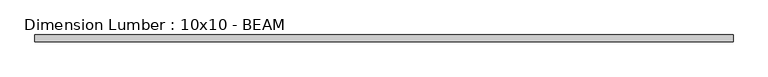
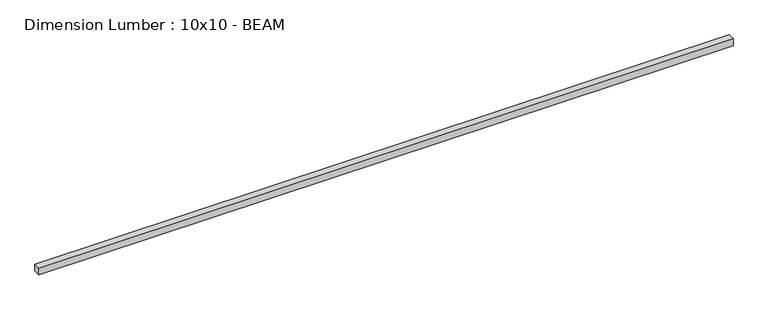
"""IFC4 building model written with IfcOpenShell, lengths in millimetres: beam geometry, Dimension Lumber : 10x10 - BEAM."""

from ifc_helpers import new_model, si_unit, frame, origin, place, context, project, spatial, polyline, outline, extrude, source, transform, mapped, element, save


def dimension_lumber_10x10_beam_a659b46f(model_context):
    return source(origin(), model_context, "Body", "SweptSolid", [
        extrude(outline(polyline([(11658.6, 117.475), (11658.6, -117.475), (-11658.6, -117.475), (-11658.6, 117.475), (11658.6, 117.475)])), frame((0.0, 0.0, -117.475), z_axis=(0.0, 0.0, 1.0), x_axis=(1.0, 0.0, 0.0)), (0.0, 0.0, 1.0), 234.95),
    ])


if __name__ == "__main__":
    model = new_model("IFC4")
    model_context = context("Model", 3, world=origin())
    ifc_project = project(units=[si_unit("LENGTHUNIT", "METRE", prefix="MILLI")], contexts=[model_context])
    site = spatial("IfcSite", under=ifc_project)
    building = spatial("IfcBuilding", under=site)
    placement = place(None, origin())
    dimension_lumber_10x10_beam_shape = dimension_lumber_10x10_beam_a659b46f(model_context)
    element("IfcBeam", 1, ObjectType="Dimension Lumber : 10x10 - BEAM", at=placement, inside=building, context=model_context, shape_type="MappedRepresentation", body=[
        mapped(dimension_lumber_10x10_beam_shape, transform((0.0, 0.0, 0.0), x_axis=(1.0, 0.0, 0.0), y_axis=(0.0, 1.0, 0.0), z_axis=(0.0, 0.0, 1.0))),
    ])
    save(model, "model.ifc")

# Revit data of these elements
# Type "Dimension Lumber : 10x10 - BEAM"
#   Assembly Code = "B10"
#   A = 0.0755556 SF
#   Length [instance default] = 5' - 0"
#   b = 0' - 9 1/4"
#   d = 0' - 9 1/4"
#   Structural Material = (4) CHARRED SISTERED 2X10s AT BEAM
# Element 1 (IfcBeam, "Dimension Lumber : 10x10 - BEAM")
#   Materials on its faces: "(4) CHARRED SISTERED 2X10s AT BEAM"
# Materials
#   "(4) CHARRED SISTERED 2X10s AT BEAM": class "Wood", colour RGB 144 144 144, transparency 0, Description = "Pinus Echinata", Cost = 0
